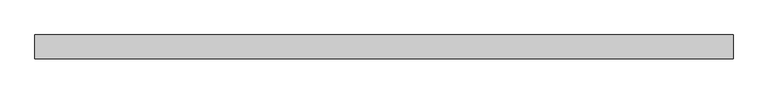
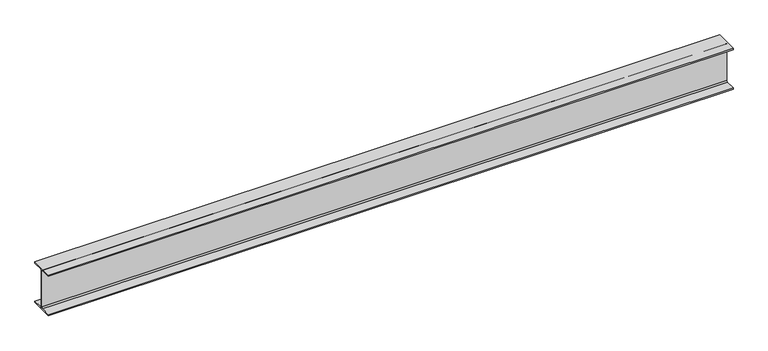
"""IFC4 building model written with IfcOpenShell, lengths in millimetres: beam geometry, Old_Steel Beam_H-KSD3502 : H_SB_ASB_H-250×125x6x9."""

from ifc_helpers import new_model, si_unit, point, frame, frame_2d, origin, place, context, project, spatial, polyline, circle_curve, trimmed, segment, composite_curve, outline, extrude, source, transform, mapped, element, save


def beam_54c8535d(model_context):
    return source(origin(), model_context, "Body", "SweptSolid", [
        extrude(outline(composite_curve([segment(polyline([(82.5, -141.5), (82.5, -151.7), (-82.5, -151.7), (-82.5, -141.5), (-11.9, -141.5)]), True, "CONTINUOUS"), segment(trimmed(circle_curve(frame_2d((-11.9, -132.6)), 8.9), [point((-11.9, -141.5))], [point((-3.0, -132.6))], True, "CARTESIAN"), True, "CONTINUOUS"), segment(polyline([(-3.0, -132.6), (-3.0, 132.6)]), True, "CONTINUOUS"), segment(trimmed(circle_curve(frame_2d((-11.9, 132.6)), 8.9), [point((-3.0, 132.6))], [point((-11.9, 141.5))], True, "CARTESIAN"), True, "CONTINUOUS"), segment(polyline([(-11.9, 141.5), (-82.5, 141.5), (-82.5, 151.7), (82.5, 151.7), (82.5, 141.5), (11.9, 141.5)]), True, "CONTINUOUS"), segment(trimmed(circle_curve(frame_2d((11.9, 132.6)), 8.9), [point((11.9, 141.5))], [point((3.0, 132.6))], True, "CARTESIAN"), True, "CONTINUOUS"), segment(polyline([(3.0, 132.6), (3.0, -132.6)]), True, "CONTINUOUS"), segment(trimmed(circle_curve(frame_2d((11.9, -132.6)), 8.9), [point((3.0, -132.6))], [point((11.9, -141.5))], True, "CARTESIAN"), True, "CONTINUOUS"), segment(polyline([(11.9, -141.5), (82.5, -141.5)]), True, "CONTINUOUS")], self_intersect=False)), frame((-2403.3634808, 0.0, 0.0), z_axis=(1.0, 0.0, 0.0), x_axis=(0.0, 1.0, 0.0)), (0.0, 0.0, 1.0), 4815.6934866),
    ])


if __name__ == "__main__":
    model = new_model("IFC4")
    model_context = context("Model", 3, world=origin())
    ifc_project = project(units=[si_unit("LENGTHUNIT", "METRE", prefix="MILLI")], contexts=[model_context])
    site = spatial("IfcSite", under=ifc_project)
    building = spatial("IfcBuilding", under=site)
    placement = place(None, origin())
    beam_shape = beam_54c8535d(model_context)
    element("IfcBeam", 1, ObjectType="Old_Steel Beam_H-KSD3502 : H_SB_ASB_H-250×125x6x9", at=placement, inside=building, context=model_context, shape_type="MappedRepresentation", body=[
        mapped(beam_shape, transform((0.0, 0.0, 0.0), x_axis=(1.0, 0.0, 0.0), y_axis=(0.0, 1.0, 0.0), z_axis=(0.0, 0.0, 1.0))),
    ])
    save(model, "model.ifc")

# Revit data of these elements
# Type "Old_Steel Beam_H-KSD3502 : H_SB_ASB_H-250×125x6x9"
#   Width = 12.5 cm
#   Web Thickness = 0.6 cm
#   Web Fillet = 1.2 cm
#   Warping Constant = 42539.8 cm⁶
#   Torsional Moment of Inertia = 7.8102 cm⁴
#   Torsional Modulus = 1.0 cm³
#   Section Area = 37.66 cm²
#   Plastic Modulus weak axis = 73.1 cm³
#   Plastic Modulus strong axis = 366.0 cm³
#   Perimeter = 0.97 m²/m
#   Nominal Weight = 29.60 kgf/m
#   Moment of Inertia weak axis = 294.00 cm⁴
#   Moment of Inertia strong axis = 4050.00 cm⁴
#   Height = 25.0 cm
#   Flange Thickness = 0.9 cm
#   Elastic Modulus weak axis = 47.0 cm³
#   Elastic Modulus strong axis = 324.0 cm³
#   Centroid Vertical = 12.5 cm
#   Centroid Horizontal = 6.25 cm
#   Length [instance default] = 1.5240 m
#   Structural Material [instance default] = Steel, 45-345
#   Assembly Code = ""
# Element 1 (IfcBeam, "Old_Steel Beam_H-KSD3502 : H_SB_ASB_H-250×125x6x9")
#   Structural Material = none
# Materials
#   "Steel, 45-345": class "Metal", colour RGB 189 187 185, transparency 0, Description = "Steel 345 MPa", Cost = 0
